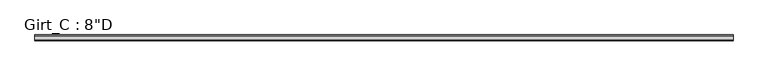
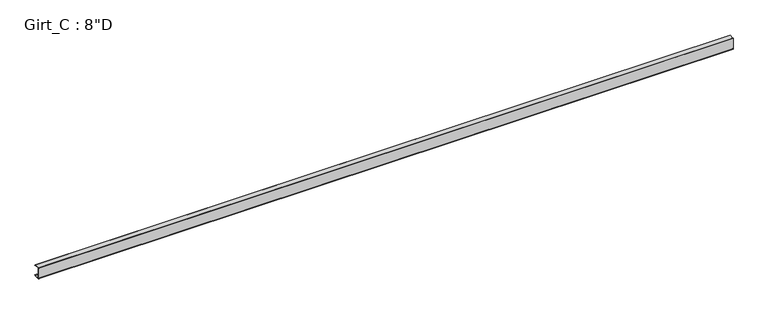
"""IFC4 building model written with IfcOpenShell, lengths in millimetres: beam geometry."""

from ifc_helpers import new_model, si_unit, point, frame, frame_2d, origin, place, context, project, spatial, polyline, circle_curve, trimmed, segment, composite_curve, outline, extrude, source, transform, mapped, element, save


def beam_58968b56(model_context):
    return source(origin(), model_context, "Body", "SweptSolid", [
        extrude(outline(composite_curve([segment(polyline([(87.5109375, 101.6), (99.7560415, 87.0068534), (97.6278742, 85.221109), (86.2154765, 98.821875), (3.3005807, 98.821875)]), True, "CONTINUOUS"), segment(trimmed(circle_curve(frame_2d((3.3741066, 96.8381931)), 1.9850441), [point((3.3005807, 98.821875))], [point((1.3890625, 96.8381931))], True, "CARTESIAN"), True, "CONTINUOUS"), segment(polyline([(1.3890625, 96.8381931), (1.3890625, -96.8389339)]), True, "CONTINUOUS"), segment(trimmed(circle_curve(frame_2d((3.3748024, -96.8389339)), 1.9857399), [point((1.3890625, -96.8389339))], [point((3.2694106, -98.821875))], True, "CARTESIAN"), True, "CONTINUOUS"), segment(polyline([(3.2694106, -98.821875), (86.2154765, -98.821875), (97.6510975, -85.1934327), (99.7792647, -86.979177), (87.5109375, -101.6), (3.3734375, -101.6)]), True, "CONTINUOUS"), segment(trimmed(circle_curve(frame_2d((3.3734375, -96.8375)), 4.7625), [point((3.3734375, -101.6))], [point((-1.3890625, -96.8375))], False, "CARTESIAN"), True, "CONTINUOUS"), segment(polyline([(-1.3890625, -96.8375), (-1.3890625, 96.8375)]), True, "CONTINUOUS"), segment(trimmed(circle_curve(frame_2d((3.3734375, 96.8375)), 4.7625), [point((-1.3890625, 96.8375))], [point((3.3734375, 101.6))], False, "CARTESIAN"), True, "CONTINUOUS"), segment(polyline([(3.3734375, 101.6), (87.5109375, 101.6)]), True, "CONTINUOUS")], self_intersect=False)), frame((-6062.8073594, 0.0, 0.0), z_axis=(1.0, 0.0, 0.0), x_axis=(0.0, 1.0, 0.0)), (0.0, 0.0, 1.0), 12223.1507188),
    ])


if __name__ == "__main__":
    model = new_model("IFC4")
    model_context = context("Model", 3, world=origin())
    ifc_project = project(units=[si_unit("LENGTHUNIT", "METRE", prefix="MILLI")], contexts=[model_context])
    site = spatial("IfcSite", under=ifc_project)
    building = spatial("IfcBuilding", under=site)
    placement = place(None, origin())
    beam_shape = beam_58968b56(model_context)
    element("IfcBeam", 1, ObjectType="Girt_C : 8\"D", at=placement, inside=building, context=model_context, shape_type="MappedRepresentation", body=[
        mapped(beam_shape, transform((0.0, 0.0, 0.0), x_axis=(1.0, 0.0, 0.0), y_axis=(0.0, 1.0, 0.0), z_axis=(0.0, 0.0, 1.0))),
    ])
    save(model, "model.ifc")

# Revit data of these elements
# Type "Girt_C : 8\"D"
#   half leg = 0' - 1 3/4"
#   Web_Thickness = 0' - 0 7/64"
#   Length [instance default] = 10' - 0"
#   Leg_1 = 0' - 3 1/2"
#   Height = 0' - 8"
#   Structural Material [instance default] = none
# Element 1 (IfcBeam, "Girt_C : 8\"D")
#   Structural Material = CEE' SECTION (8.0x3.5C - SEE STRUCT. DWGS)
#   Materials on its faces: "CEE' SECTION (8.0x3.5C - SEE STRUCT. DWGS)"
# Materials
#   "CEE' SECTION (8.0x3.5C - SEE STRUCT. DWGS)": class "Metal", colour RGB 137 146 153, transparency 0, Description = "Steel, mill finish", Cost = 0
